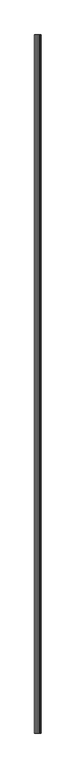
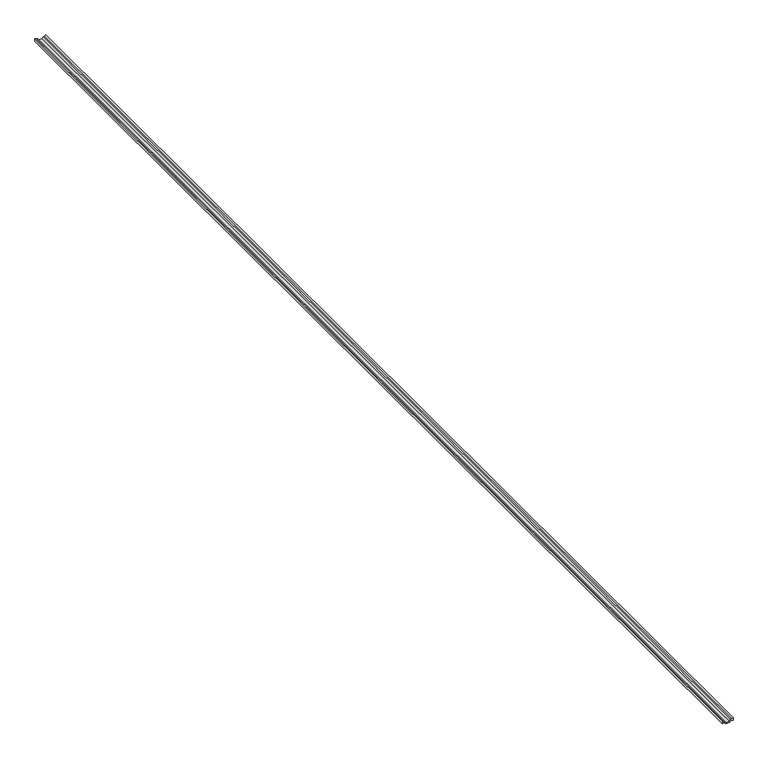
"""IFC4 building model written with IfcOpenShell, lengths in millimetres: proxy geometry, Door frame14:Door frame013:296498 : Door frame14:Door frame013:296498."""

from ifc_helpers import new_model, si_unit, frame, origin, place, context, project, spatial, polyline, outline, extrude, source, transform, mapped, element, save


def generic_models_6b17c4ba(model_context):
    return source(origin(), model_context, "Body", "SweptSolid", [
        extrude(outline(polyline([(36593.6518099, 20329.9993083), (36596.1835829, 20331.7720748), (36596.1835829, 20333.3106739), (36595.1059519, 20335.7310727), (36599.8429954, 20335.7310727), (36598.3174519, 20333.0887538), (36598.3174519, 20331.3129866), (36595.2518099, 20329.166401), (36595.2518099, 20323.8176572), (36598.3174519, 20321.6710716), (36598.3174519, 20319.8953044), (36599.8429954, 20317.2529855), (36595.1059519, 20317.2529855), (36596.1835829, 20319.6733843), (36596.1835829, 20321.2119834), (36593.6518099, 20322.9847499), (36593.6518099, 20329.9993083)])), frame((0.0, -774.5581156, 0.0), z_axis=(0.0, 1.0, 0.0), x_axis=(0.0, 0.0, 1.0)), (0.0, 0.0, 1.0), 1999.85),
    ])


if __name__ == "__main__":
    model = new_model("IFC4")
    model_context = context("Model", 3, world=origin())
    ifc_project = project(units=[si_unit("LENGTHUNIT", "METRE", prefix="MILLI")], contexts=[model_context])
    site = spatial("IfcSite", under=ifc_project)
    building = spatial("IfcBuilding", under=site)
    placement = place(None, origin())
    generic_models_shape = generic_models_6b17c4ba(model_context)
    element("IfcBuildingElementProxy", 1, Name="Door frame14:Door frame013:296498 : Door frame14:Door frame013:296498", ObjectType="Door frame14:Door frame013:296498 : Door frame14:Door frame013:296498", at=placement, inside=building, context=model_context, shape_type="MappedRepresentation", body=[
        mapped(generic_models_shape, transform((0.0, 0.0, 0.0), x_axis=(1.0, 0.0, 0.0), y_axis=(0.0, 1.0, 0.0), z_axis=(0.0, 0.0, 1.0))),
    ])
    save(model, "model.ifc")

# Revit data of these elements
# Type "Door frame14:Door frame013:296498 : Door frame14:Door frame013:296498"
#   NameOverride = "Door frame14:Door frame013:296498"
#   ObjectTypeOverride = "Door frame14:Door frame013"
#   Reference = "Door frame013"
#   Category = "Generic Models"
#   Tag = "296498"
# Element 1 (IfcBuildingElementProxy, "Door frame14:Door frame013:296498 : Door frame14:Door frame013:296498")
#   Materials on its faces: "FLEETWOOD SERIES T-3200 SINGLE SWING DOOR FRAME"
# Materials
#   "FLEETWOOD SERIES T-3200 SINGLE SWING DOOR FRAME": class "Unassigned", colour RGB 128 128 128, transparency 0, Cost = 0
